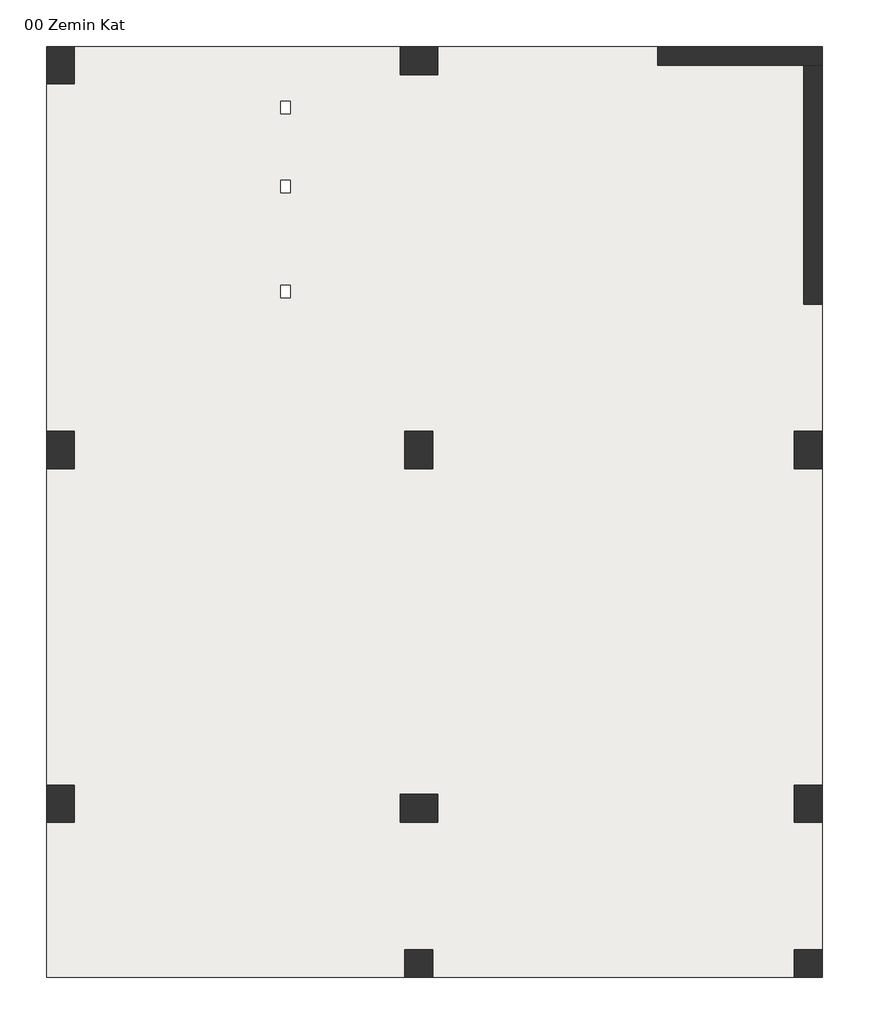
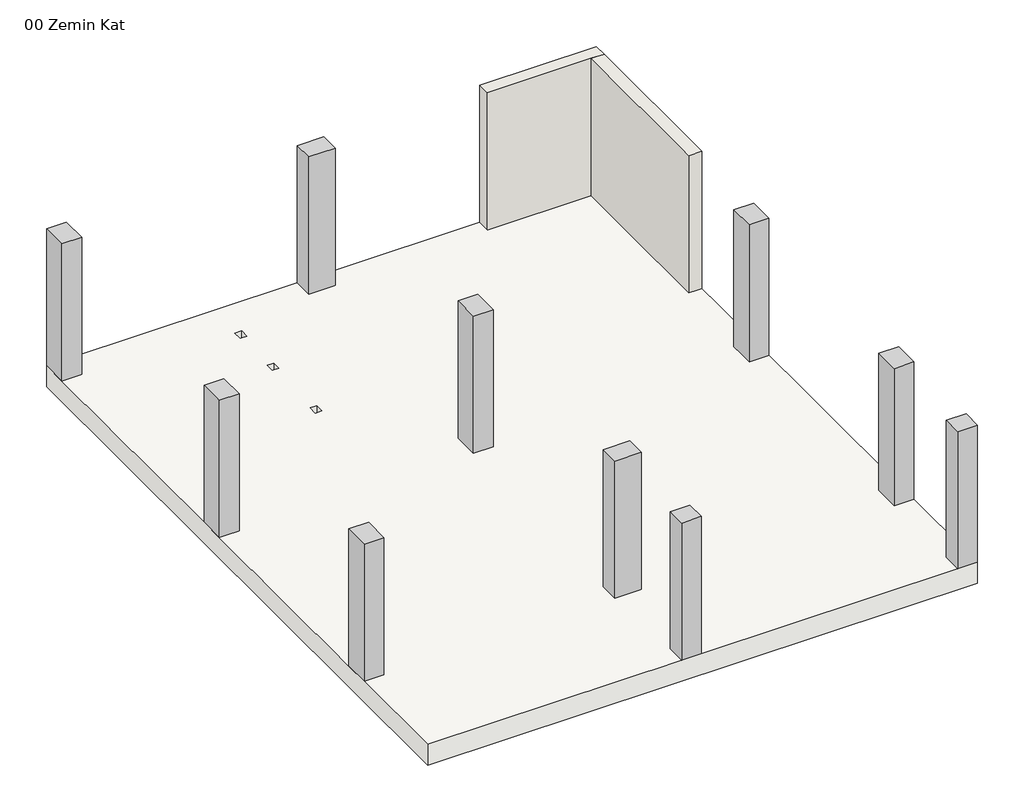
# One storey: 10 columns, 2 walls, 1 slab.
"""IFC4 building model written with IfcOpenShell, lengths in millimetres."""

from ifc_helpers import new_model, si_unit, frame, origin, place, context, project, spatial, polyline, outline, extrude, faceted_brep, element, save

model = new_model("IFC4")

# Units and contexts
model_context = context("Model", 3, world=origin())
ifc_project = project(units=[si_unit("LENGTHUNIT", "METRE", prefix="MILLI")], contexts=[model_context])

# Site, building, storey
site = spatial("IfcSite", under=ifc_project)
building = spatial("IfcBuilding", under=site)
storey = spatial("IfcBuildingStorey", under=building, Name="00 Zemin Kat", Elevation=93780.0)

# Columns
placement = place(None, origin())
element("IfcColumn", 1, ObjectType="M_Concrete-Rectangular-Column : 45x60cm Kolon", at=placement, inside=storey, context=model_context, shape_type="SweptSolid", body=[
    extrude(outline(polyline([(0.0, 14400.0), (0.0, 15000.0), (450.0, 15000.0), (450.0, 14400.0), (0.0, 14400.0)])), frame((0.0, 0.0, 93780.0), z_axis=(0.0, 0.0, 1.0), x_axis=(1.0, 0.0, 0.0)), (0.0, 0.0, 1.0), 3300.0),
])
element("IfcColumn", 2, ObjectType="M_Concrete-Rectangular-Column : 45x60cm Kolon", at=placement, inside=storey, context=model_context, shape_type="SweptSolid", body=[
    extrude(outline(polyline([(5700.0, 14999.2150597), (6300.0, 14999.2150597), (6300.0, 14549.2150597), (5700.0, 14549.2150597), (5700.0, 14999.2150597)])), frame((0.0, 0.0, 93780.0), z_axis=(0.0, 0.0, 1.0), x_axis=(1.0, 0.0, 0.0)), (0.0, 0.0, 1.0), 3300.0),
])
element("IfcColumn", 3, ObjectType="M_Concrete-Rectangular-Column : 45x60cm Kolon", at=placement, inside=storey, context=model_context, shape_type="SweptSolid", body=[
    extrude(outline(polyline([(450.0, 8800.0), (450.0, 8200.0), (0.0, 8200.0), (0.0, 8800.0), (450.0, 8800.0)])), frame((0.0, 0.0, 93780.0), z_axis=(0.0, 0.0, 1.0), x_axis=(1.0, 0.0, 0.0)), (0.0, 0.0, 1.0), 3300.0),
])
element("IfcColumn", 4, ObjectType="M_Concrete-Rectangular-Column : 45x60cm Kolon", at=placement, inside=storey, context=model_context, shape_type="SweptSolid", body=[
    extrude(outline(polyline([(6225.0, 8800.0), (6225.0, 8200.0), (5775.0, 8200.0), (5775.0, 8800.0), (6225.0, 8800.0)])), frame((0.0, 0.0, 93780.0), z_axis=(0.0, 0.0, 1.0), x_axis=(1.0, 0.0, 0.0)), (0.0, 0.0, 1.0), 3300.0),
])
element("IfcColumn", 5, ObjectType="M_Concrete-Rectangular-Column : 45x60cm Kolon", at=placement, inside=storey, context=model_context, shape_type="SweptSolid", body=[
    extrude(outline(polyline([(12494.8117928, 8800.0), (12494.8117928, 8200.0), (12044.8117928, 8200.0), (12044.8117928, 8800.0), (12494.8117928, 8800.0)])), frame((0.0, 0.0, 93780.0), z_axis=(0.0, 0.0, 1.0), x_axis=(1.0, 0.0, 0.0)), (0.0, 0.0, 1.0), 3300.0),
])
element("IfcColumn", 6, ObjectType="M_Concrete-Rectangular-Column : 45x60cm Kolon", at=placement, inside=storey, context=model_context, shape_type="SweptSolid", body=[
    extrude(outline(polyline([(12500.0, 3100.0), (12500.0, 2500.0), (12050.0, 2500.0), (12050.0, 3100.0), (12500.0, 3100.0)])), frame((0.0, 0.0, 93780.0), z_axis=(0.0, 0.0, 1.0), x_axis=(1.0, 0.0, 0.0)), (0.0, 0.0, 1.0), 3300.0),
])
element("IfcColumn", 7, ObjectType="M_Concrete-Rectangular-Column : 45x60cm Kolon", at=placement, inside=storey, context=model_context, shape_type="SweptSolid", body=[
    extrude(outline(polyline([(450.0, 3100.0), (450.0, 2500.0), (0.0, 2500.0), (0.0, 3100.0), (450.0, 3100.0)])), frame((0.0, 0.0, 93780.0), z_axis=(0.0, 0.0, 1.0), x_axis=(1.0, 0.0, 0.0)), (0.0, 0.0, 1.0), 3300.0),
])
element("IfcColumn", 8, ObjectType="M_Concrete-Rectangular-Column : 45x60cm Kolon", at=placement, inside=storey, context=model_context, shape_type="SweptSolid", body=[
    extrude(outline(polyline([(5700.0, 2950.0), (6300.0, 2950.0), (6300.0, 2500.0), (5700.0, 2500.0), (5700.0, 2950.0)])), frame((0.0, 0.0, 93780.0), z_axis=(0.0, 0.0, 1.0), x_axis=(1.0, 0.0, 0.0)), (0.0, 0.0, 1.0), 3300.0),
])
element("IfcColumn", 9, ObjectType="M_Concrete-Rectangular-Column : 45x45cm Kolon", at=placement, inside=storey, context=model_context, shape_type="SweptSolid", body=[
    extrude(outline(polyline([(6225.0, 450.0), (6225.0, 0.0), (5775.0, 0.0), (5775.0, 450.0), (6225.0, 450.0)])), frame((0.0, 0.0, 93780.0), z_axis=(0.0, 0.0, 1.0), x_axis=(1.0, 0.0, 0.0)), (0.0, 0.0, 1.0), 3300.0),
])
element("IfcColumn", 10, ObjectType="M_Concrete-Rectangular-Column : 45x45cm Kolon", at=placement, inside=storey, context=model_context, shape_type="SweptSolid", body=[
    extrude(outline(polyline([(12500.0, 450.0), (12500.0, 0.0), (12050.0, 0.0), (12050.0, 450.0), (12500.0, 450.0)])), frame((0.0, 0.0, 93780.0), z_axis=(0.0, 0.0, 1.0), x_axis=(1.0, 0.0, 0.0)), (0.0, 0.0, 1.0), 3300.0),
])

# Slab
element("IfcSlab", 11, ObjectType="50cm Döşeme", at=placement, inside=storey, context=model_context, shape_type="Brep", body=[
    faceted_brep([(12500.0, 15000.0, 93280.0), (12500.0, 0.0, 93280.0), (0.0, 0.0, 93280.0), (0.0, 15000.0, 93280.0), (3775.0, 13920.0, 93280.0), (3925.0, 13920.0, 93280.0), (3925.0, 14120.0, 93280.0), (3775.0, 14120.0, 93280.0), (3775.0, 12646.5789726, 93280.0), (3925.0, 12646.5789726, 93280.0), (3925.0, 12846.5789726, 93280.0), (3775.0, 12846.5789726, 93280.0), (3775.0, 10954.975, 93280.0), (3925.0, 10954.975, 93280.0), (3925.0, 11154.975, 93280.0), (3775.0, 11154.975, 93280.0), (12500.0, 15000.0, 93780.0), (450.0, 15000.0, 93780.0), (0.0, 15000.0, 93780.0), (0.0, 14400.0, 93780.0), (0.0, 8800.0, 93780.0), (0.0, 8200.0, 93780.0), (0.0, 3100.0, 93780.0), (0.0, 2500.0, 93780.0), (0.0, 0.0, 93780.0), (5775.0, 0.0, 93780.0), (6225.0, 0.0, 93780.0), (12050.0, 0.0, 93780.0), (12500.0, 0.0, 93780.0), (12500.0, 450.0, 93780.0), (12500.0, 2500.0, 93780.0), (12500.0, 3100.0, 93780.0), (3775.0, 13920.0, 93780.0), (3775.0, 14120.0, 93780.0), (3925.0, 14120.0, 93780.0), (3925.0, 13920.0, 93780.0), (3775.0, 12646.5789726, 93780.0), (3775.0, 12846.5789726, 93780.0), (3925.0, 12846.5789726, 93780.0), (3925.0, 12646.5789726, 93780.0), (3775.0, 10954.975, 93780.0), (3775.0, 11154.975, 93780.0), (3925.0, 11154.975, 93780.0), (3925.0, 10954.975, 93780.0)], [[[0, 1, 2, 3], [4, 5, 6, 7], [8, 9, 10, 11], [12, 13, 14, 15]], [[16, 17, 18, 19, 20, 21, 22, 23, 24, 25, 26, 27, 28, 29, 30, 31], [32, 33, 34, 35], [36, 37, 38, 39], [40, 41, 42, 43]], [[1, 0, 16, 31, 30, 29, 28]], [[2, 1, 28, 27, 26, 25, 24]], [[3, 2, 24, 23, 22, 21, 20, 19, 18]], [[0, 3, 18, 17, 16]], [[5, 4, 32, 35]], [[6, 5, 35, 34]], [[7, 6, 34, 33]], [[4, 7, 33, 32]], [[9, 8, 36, 39]], [[10, 9, 39, 38]], [[11, 10, 38, 37]], [[8, 11, 37, 36]], [[13, 12, 40, 43]], [[14, 13, 43, 42]], [[15, 14, 42, 41]], [[12, 15, 41, 40]]]),
])

# Walls
element("IfcWall", 12, ObjectType="30cm Perde Duvar", at=placement, inside=storey, context=model_context, shape_type="Brep", body=[
    faceted_brep([(9850.0, 14700.0, 93780.0), (12200.0, 14700.0, 93780.0), (12500.0, 14700.0, 93780.0), (12500.0, 14700.0, 97080.0), (12200.0, 14700.0, 97080.0), (9850.0, 14700.0, 97080.0), (9850.0, 14700.0, 96680.0), (9850.0, 15000.0, 93780.0), (9850.0, 15000.0, 96680.0), (9850.0, 15000.0, 97080.0), (12500.0, 15000.0, 97080.0), (12500.0, 15000.0, 93780.0)], [[[0, 1, 2, 3, 4, 5, 6]], [[7, 8, 9, 10, 11]], [[2, 1, 0, 7, 11]], [[0, 6, 5, 9, 8, 7]], [[3, 2, 11, 10]], [[5, 4, 3, 10, 9]]]),
])
element("IfcWall", 13, ObjectType="30cm Perde Duvar", at=placement, inside=storey, context=model_context, shape_type="Brep", body=[
    faceted_brep([(12200.0, 14700.0, 93780.0), (12200.0, 10850.0, 93780.0), (12200.0, 10850.0, 96680.0), (12200.0, 10850.0, 97080.0), (12200.0, 14700.0, 97080.0), (12500.0, 14700.0, 93780.0), (12500.0, 14700.0, 97080.0), (12500.0, 10850.0, 97080.0), (12500.0, 10850.0, 96680.0), (12500.0, 10850.0, 93780.0)], [[[0, 1, 2, 3, 4]], [[5, 6, 7, 8, 9]], [[1, 0, 5, 9]], [[3, 2, 1, 9, 8, 7]], [[0, 4, 6, 5]], [[4, 3, 7, 6]]]),
])

save(model, "model.ifc")

# Revit data of these elements
# Project information
#   Project Issue Date = "Issue Date"
#   Project Status = "Project Status"
#   Client Name = "Owner"
#   Project Address = "Enter address here"
#   Project Name = "Project Name"
#   Project Number = "0001"
# Grids (mm)
#   "1": line (0, -1446.356) -> (0, 16597.874)
#   "2": line (6000, -1446.356) -> (6000, 16597.874)
#   "3": line (12500, -1446.356) -> (12500, 16597.874)
#   "A": line (-3259.789, 0) -> (14827.9, 0)
#   "B": line (-3259.789, 2500) -> (14827.9, 2500)
#   "C": line (-3259.789, 8500) -> (14827.9, 8500)
#   "D": line (-3259.789, 15000) -> (14827.9, 15000)
# Type "M_Concrete-Rectangular-Column : 45x60cm Kolon"
#   b = 45.00 cm
#   h = 60.00 cm
#   Structural Material [instance default] = Concrete, Cast-in-Place gray
# Type "M_Concrete-Rectangular-Column : 45x45cm Kolon"
#   b = 45.00 cm
#   h = 45.00 cm
#   Structural Material [instance default] = Concrete, Cast-in-Place gray
# Type "50cm Döşeme"
#   Function = 0
#   Layers, outside or top first: 50.00 cm "Concrete, Cast In Situ" (function 1)
# Type "30cm Perde Duvar"
#   Layers, outside or top first: 30.00 cm "Concrete, Cast In Situ" (function 1)
# Elements 1, 2, 3, 4, 5, 6, 7, 8 (IfcColumn, "M_Concrete-Rectangular-Column : 45x60cm Kolon")
#   Comments = ""
#   Structural Material = Concrete, Cast-in-Place gray
#   Phase Created = New Construction
#   Materials on its faces: "Concrete, Cast-in-Place gray"
# Elements 9, 10 (IfcColumn, "M_Concrete-Rectangular-Column : 45x45cm Kolon")
#   Comments = ""
#   Structural Material = Concrete, Cast-in-Place gray
#   Phase Created = New Construction
#   Materials on its faces: "Concrete, Cast-in-Place gray"
# Element 11 (IfcSlab, "50cm Döşeme")
#   Height Offset From Level = 0.00 cm
#   built-in parameter 1001954 = 1
#   Phase Created = New Construction
#   Materials on its faces: "Concrete, Cast In Situ"
# Elements 12, 13 (IfcWall, "30cm Perde Duvar")
#   Comments = ""
#   Top Offset = 0.00 cm
#   Base Offset = 0.00 cm
#   wall height = 330.00 cm
#   Phase Created = New Construction
#   Base Constraint = 00 Zemin Kat
#   Top Constraint = 01 Birinci Kat
#   Materials on its faces: "Concrete, Cast In Situ"
# Materials
#   "Concrete, Cast-in-Place gray": class "Concrete", colour RGB 192 192 192, transparency 0, Description = "Cast-in-place concrete", Cost = 0
#   "Concrete, Cast In Situ": class "Concrete", colour RGB 192 192 192, transparency 0, Description = "physical material", Cost = 0
